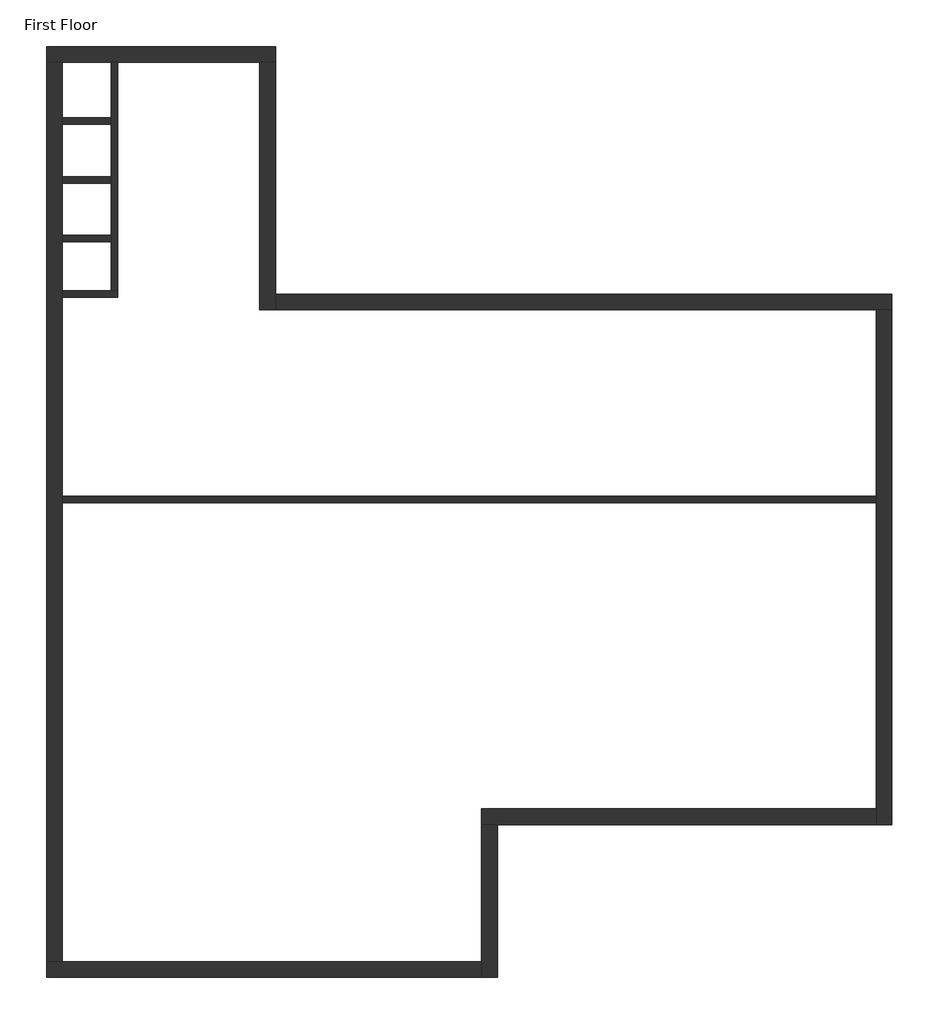
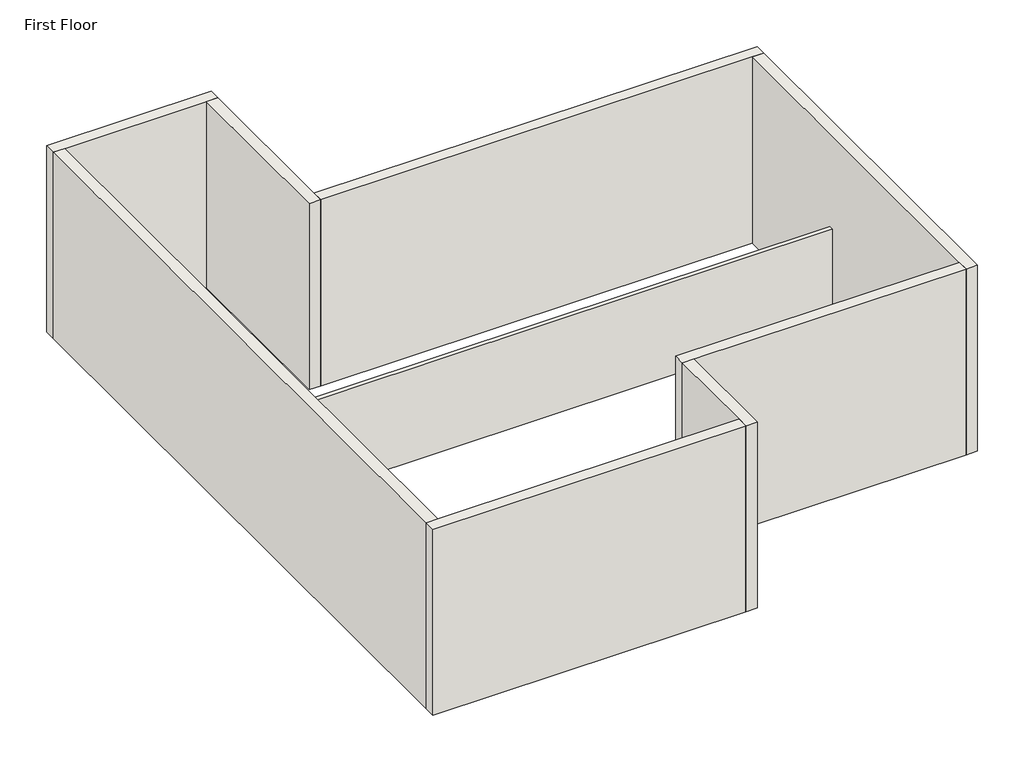
# One storey: 14 walls.
"""IFC4 building model written with IfcOpenShell, lengths in millimetres."""

from ifc_helpers import new_model, si_unit, origin, origin_with_axes, place, context, project, spatial, polyline, outline, extrude, faceted_brep, element, save

model = new_model("IFC4")

# Units and contexts
model_context = context("Model", 3, world=origin())
ifc_project = project(units=[si_unit("LENGTHUNIT", "METRE", prefix="MILLI")], contexts=[model_context])

# Site, building, storey
site = spatial("IfcSite", under=ifc_project)
building = spatial("IfcBuilding", under=site)
storey = spatial("IfcBuildingStorey", under=building, Name="First Floor", Elevation=0.0)

# Walls
placement = place(None, origin())
element("IfcWall", 1, ObjectType="Exterior - Brick on Wood Stud", at=placement, inside=storey, context=model_context, shape_type="Brep", body=[
    faceted_brep([(-11220.7128554, 8382.2404543, 0.0), (-10938.1378554, 8382.2404543, 0.0), (-10069.7753554, 8382.2404543, 0.0), (-9955.4753554, 8382.2404543, 0.0), (-7421.8253554, 8382.2404543, 0.0), (-7139.2503554, 8382.2404543, 0.0), (-7139.2503554, 8382.2404543, 4876.8), (-7421.8253554, 8382.2404543, 4876.8), (-10938.1378554, 8382.2404543, 4876.8), (-11220.7128554, 8382.2404543, 4876.8), (-11220.7128554, 8664.8154543, 0.0), (-11220.7128554, 8664.8154543, 4876.8), (-7139.2503554, 8664.8154543, 4876.8), (-7139.2503554, 8664.8154543, 0.0)], [[[0, 1, 2, 3, 4, 5, 6, 7, 8, 9]], [[10, 11, 12, 13]], [[5, 4, 3, 2, 1, 0, 10, 13]], [[9, 8, 7, 6, 12, 11]], [[6, 5, 13, 12]], [[0, 9, 11, 10]]]),
])
element("IfcWall", 2, ObjectType="Exterior - Brick on Wood Stud", at=placement, inside=storey, context=model_context, shape_type="Brep", body=[
    faceted_brep([(-7421.8253554, 8382.2404543, 0.0), (-7421.8253554, 3973.7529543, 0.0), (-7421.8253554, 3973.7529543, 4876.8), (-7421.8253554, 8382.2404543, 4876.8), (-7139.2503554, 8382.2404543, 0.0), (-7139.2503554, 8382.2404543, 4876.8), (-7139.2503554, 4256.3279543, 4876.8), (-7139.2503554, 3973.7529543, 4876.8), (-7139.2503554, 3973.7529543, 0.0), (-7139.2503554, 4256.3279543, 0.0)], [[[0, 1, 2, 3]], [[4, 5, 6, 7, 8, 9]], [[1, 0, 4, 9, 8]], [[3, 2, 7, 6, 5]], [[0, 3, 5, 4]], [[2, 1, 8, 7]]]),
])
element("IfcWall", 3, ObjectType="Exterior - Brick on Wood Stud", at=placement, inside=storey, context=model_context, shape_type="Brep", body=[
    faceted_brep([(-7139.2503554, 3973.7529543, 0.0), (3562.0871446, 3973.7529543, 0.0), (3844.6621446, 3973.7529543, 0.0), (3844.6621446, 3973.7529543, 4876.8), (3562.0871446, 3973.7529543, 4876.8), (-7139.2503554, 3973.7529543, 4876.8), (-7139.2503554, 4256.3279543, 0.0), (-7139.2503554, 4256.3279543, 4876.8), (3844.6621446, 4256.3279543, 4876.8), (3844.6621446, 4256.3279543, 0.0)], [[[0, 1, 2, 3, 4, 5]], [[6, 7, 8, 9]], [[2, 1, 0, 6, 9]], [[5, 4, 3, 8, 7]], [[0, 5, 7, 6]], [[3, 2, 9, 8]]]),
])
element("IfcWall", 4, ObjectType="Exterior - Brick on Wood Stud", at=placement, inside=storey, context=model_context, shape_type="Brep", body=[
    faceted_brep([(3562.0871446, 3973.7529543, 0.0), (3562.0871446, 655.8779543, 0.0), (3562.0871446, 541.5779543, 0.0), (3562.0871446, -4909.8970457, 0.0), (3562.0871446, -5192.4720457, 0.0), (3562.0871446, -5192.4720457, 4876.8), (3562.0871446, -4909.8970457, 4876.8), (3562.0871446, 3973.7529543, 4876.8), (3844.6621446, 3973.7529543, 0.0), (3844.6621446, 3973.7529543, 4876.8), (3844.6621446, -5192.4720457, 4876.8), (3844.6621446, -5192.4720457, 0.0)], [[[0, 1, 2, 3, 4, 5, 6, 7]], [[8, 9, 10, 11]], [[4, 3, 2, 1, 0, 8, 11]], [[7, 6, 5, 10, 9]], [[0, 7, 9, 8]], [[5, 4, 11, 10]]]),
])
element("IfcWall", 5, ObjectType="Exterior - Brick on Wood Stud", at=placement, inside=storey, context=model_context, shape_type="Brep", body=[
    faceted_brep([(3562.0871446, -4909.8970457, 0.0), (-3470.5378554, -4909.8970457, 0.0), (-3470.5378554, -4909.8970457, 4876.8), (3562.0871446, -4909.8970457, 4876.8), (3562.0871446, -5192.4720457, 0.0), (3562.0871446, -5192.4720457, 4876.8), (-3187.9628554, -5192.4720457, 4876.8), (-3470.5378554, -5192.4720457, 4876.8), (-3470.5378554, -5192.4720457, 0.0), (-3187.9628554, -5192.4720457, 0.0)], [[[0, 1, 2, 3]], [[4, 5, 6, 7, 8, 9]], [[1, 0, 4, 9, 8]], [[3, 2, 7, 6, 5]], [[0, 3, 5, 4]], [[2, 1, 8, 7]]]),
])
element("IfcWall", 6, ObjectType="Exterior - Brick on Wood Stud", at=placement, inside=storey, context=model_context, shape_type="Brep", body=[
    faceted_brep([(-3470.5378554, -5192.4720457, 0.0), (-3470.5378554, -7630.8720457, 0.0), (-3470.5378554, -7913.4470457, 0.0), (-3470.5378554, -7913.4470457, 4876.8), (-3470.5378554, -7630.8720457, 4876.8), (-3470.5378554, -5192.4720457, 4876.8), (-3187.9628554, -5192.4720457, 0.0), (-3187.9628554, -5192.4720457, 4876.8), (-3187.9628554, -7913.4470457, 4876.8), (-3187.9628554, -7913.4470457, 0.0)], [[[0, 1, 2, 3, 4, 5]], [[6, 7, 8, 9]], [[2, 1, 0, 6, 9]], [[5, 4, 3, 8, 7]], [[0, 5, 7, 6]], [[3, 2, 9, 8]]]),
])
element("IfcWall", 7, ObjectType="Exterior - Brick on Wood Stud", at=placement, inside=storey, context=model_context, shape_type="Brep", body=[
    faceted_brep([(-3470.5378554, -7630.8720457, 0.0), (-10938.1378554, -7630.8720457, 0.0), (-11220.7128554, -7630.8720457, 0.0), (-11220.7128554, -7630.8720457, 4876.8), (-10938.1378554, -7630.8720457, 4876.8), (-3470.5378554, -7630.8720457, 4876.8), (-3470.5378554, -7913.4470457, 0.0), (-3470.5378554, -7913.4470457, 4876.8), (-11220.7128554, -7913.4470457, 4876.8), (-11220.7128554, -7913.4470457, 0.0)], [[[0, 1, 2, 3, 4, 5]], [[6, 7, 8, 9]], [[2, 1, 0, 6, 9]], [[5, 4, 3, 8, 7]], [[0, 5, 7, 6]], [[3, 2, 9, 8]]]),
])
element("IfcWall", 8, ObjectType="Exterior - Brick on Wood Stud", at=placement, inside=storey, context=model_context, shape_type="Brep", body=[
    faceted_brep([(-10938.1378554, -7630.8720457, 0.0), (-10938.1378554, 541.5779543, 0.0), (-10938.1378554, 655.8779543, 0.0), (-10938.1378554, 4199.1779543, 0.0), (-10938.1378554, 4313.4779543, 0.0), (-10938.1378554, 5187.7935793, 0.0), (-10938.1378554, 5302.0935793, 0.0), (-10938.1378554, 6233.5592043, 0.0), (-10938.1378554, 6347.8592043, 0.0), (-10938.1378554, 7279.3248293, 0.0), (-10938.1378554, 7393.6248293, 0.0), (-10938.1378554, 8382.2404543, 0.0), (-10938.1378554, 8382.2404543, 4876.8), (-10938.1378554, -7630.8720457, 4876.8), (-11220.7128554, -7630.8720457, 0.0), (-11220.7128554, -7630.8720457, 4876.8), (-11220.7128554, 8382.2404543, 4876.8), (-11220.7128554, 8382.2404543, 0.0)], [[[0, 1, 2, 3, 4, 5, 6, 7, 8, 9, 10, 11, 12, 13]], [[14, 15, 16, 17]], [[11, 10, 9, 8, 7, 6, 5, 4, 3, 2, 1, 0, 14, 17]], [[13, 12, 16, 15]], [[0, 13, 15, 14]], [[12, 11, 17, 16]]]),
])
element("IfcWall", 9, ObjectType="Interior - 4 1/2\" Partition", at=placement, inside=storey, context=model_context, shape_type="SweptSolid", body=[
    extrude(outline(polyline([(3562.0871446, 541.5779543), (-10938.1378554, 541.5779543), (-10938.1378554, 655.8779543), (3562.0871446, 655.8779543), (3562.0871446, 541.5779543)])), origin_with_axes(), (0.0, 0.0, 1.0), 2438.4),
])
element("IfcWall", 10, ObjectType="Interior - 4 1/2\" Partition", at=placement, inside=storey, context=model_context, shape_type="Brep", body=[
    faceted_brep([(-10938.1378554, 4199.1779543, 0.0), (-9955.4753554, 4199.1779543, 0.0), (-9955.4753554, 4199.1779543, 2438.4), (-10938.1378554, 4199.1779543, 2438.4), (-10938.1378554, 4313.4779543, 0.0), (-10938.1378554, 4313.4779543, 2438.4), (-10069.7753554, 4313.4779543, 2438.4), (-9955.4753554, 4313.4779543, 2438.4), (-9955.4753554, 4313.4779543, 0.0), (-10069.7753554, 4313.4779543, 0.0)], [[[0, 1, 2, 3]], [[4, 5, 6, 7, 8, 9]], [[1, 0, 4, 9, 8]], [[3, 2, 7, 6, 5]], [[0, 3, 5, 4]], [[2, 1, 8, 7]]]),
])
element("IfcWall", 11, ObjectType="Interior - 4 1/2\" Partition", at=placement, inside=storey, context=model_context, shape_type="Brep", body=[
    faceted_brep([(-9955.4753554, 4313.4779543, 0.0), (-9955.4753554, 8382.2404543, 0.0), (-9955.4753554, 8382.2404543, 2438.4), (-9955.4753554, 4313.4779543, 2438.4), (-10069.7753554, 4313.4779543, 0.0), (-10069.7753554, 4313.4779543, 2438.4), (-10069.7753554, 5187.7935793, 2438.4), (-10069.7753554, 5302.0935793, 2438.4), (-10069.7753554, 6233.5592043, 2438.4), (-10069.7753554, 6347.8592043, 2438.4), (-10069.7753554, 7279.3248293, 2438.4), (-10069.7753554, 7393.6248293, 2438.4), (-10069.7753554, 8382.2404543, 2438.4), (-10069.7753554, 8382.2404543, 0.0), (-10069.7753554, 7393.6248293, 0.0), (-10069.7753554, 7279.3248293, 0.0), (-10069.7753554, 6347.8592043, 0.0), (-10069.7753554, 6233.5592043, 0.0), (-10069.7753554, 5302.0935793, 0.0), (-10069.7753554, 5187.7935793, 0.0)], [[[0, 1, 2, 3]], [[4, 5, 6, 7, 8, 9, 10, 11, 12, 13, 14, 15, 16, 17, 18, 19]], [[1, 0, 4, 19, 18, 17, 16, 15, 14, 13]], [[3, 2, 12, 11, 10, 9, 8, 7, 6, 5]], [[0, 3, 5, 4]], [[2, 1, 13, 12]]]),
])
element("IfcWall", 12, ObjectType="Interior - 4 1/2\" Partition", at=placement, inside=storey, context=model_context, shape_type="SweptSolid", body=[
    extrude(outline(polyline([(-10069.7753554, 5187.7935793), (-10938.1378554, 5187.7935793), (-10938.1378554, 5302.0935793), (-10069.7753554, 5302.0935793), (-10069.7753554, 5187.7935793)])), origin_with_axes(), (0.0, 0.0, 1.0), 2438.4),
])
element("IfcWall", 13, ObjectType="Interior - 4 1/2\" Partition", at=placement, inside=storey, context=model_context, shape_type="SweptSolid", body=[
    extrude(outline(polyline([(-10069.7753554, 6233.5592043), (-10938.1378554, 6233.5592043), (-10938.1378554, 6347.8592043), (-10069.7753554, 6347.8592043), (-10069.7753554, 6233.5592043)])), origin_with_axes(), (0.0, 0.0, 1.0), 2438.4),
])
element("IfcWall", 14, ObjectType="Interior - 4 1/2\" Partition", at=placement, inside=storey, context=model_context, shape_type="SweptSolid", body=[
    extrude(outline(polyline([(-10069.7753554, 7279.3248293), (-10938.1378554, 7279.3248293), (-10938.1378554, 7393.6248293), (-10069.7753554, 7393.6248293), (-10069.7753554, 7279.3248293)])), origin_with_axes(), (0.0, 0.0, 1.0), 2438.4),
])

save(model, "model.ifc")

# Revit data of these elements
# Project information
#   Project Issue Date = "Issue Date"
#   Project Status = "Project Status"
#   Client Name = "Owner"
#   Project Address = "Enter address here"
#   Project Name = "Project Name"
#   Project Number = "Project Number"
# Grids (mm)
#   "1": line (-10938.138, -13775.472) -> (-10938.138, 9288.695)
#   "2": line (-7280.538, -13775.472) -> (-7280.538, 9288.695)
#   "3": line (-3470.538, -13775.472) -> (-3470.538, 9288.695)
#   "4": line (187.062, -13775.472) -> (187.062, 9288.695)
#   "5": line (3844.662, -13775.472) -> (3844.662, 9288.695)
#   "B": line (6207.412, 4256.328) -> (-13740.722, 4256.328)
#   "C": line (6207.412, 598.728) -> (-13740.722, 598.728)
#   "D": line (6207.412, -3058.872) -> (-13740.722, -3058.872)
#   "D.1": line (6207.412, -5192.472) -> (-13740.722, -5192.472)
#   "E": line (6207.412, -7630.872) -> (-13740.722, -7630.872)
#   "F": line (6207.412, -11898.072) -> (-13740.722, -11898.072)
#   "A": line (6207.412, 7913.928) -> (-13740.722, 7913.928)
# Type "Exterior - Brick on Wood Stud"
#   Assembly Code = "B2010158"
#   Layers, outside or top first: 0' - 3 5/8" "Brick, Common" (function 4); 0' - 1" "Air" (function 3); 0' - 0" "Air Infiltration Barrier" (function 100); 0' - 0 1/2" "Plywood, Sheathing" (function 2); 0' - 5 1/2" "Softwood, Lumber" (function 1); 0' - 0" "Vapor Retarder" (function 100); 0' - 0 1/2" "Gypsum Wall Board" (function 5)
# Type "Interior - 4 1/2\" Partition"
#   Assembly Code = "C1010145"
#   Layers, outside or top first: 0' - 0 1/2" "Gypsum Wall Board" (function 5); 0' - 3 1/2" "Softwood, Lumber" (function 1); 0' - 0 1/2" "Gypsum Wall Board" (function 5)
# Element 1 (IfcWall, "Exterior - Brick on Wood Stud")
#   Top Offset = 0' - 0"
#   Base Offset = 0' - 0"
#   wall height = 16' - 0"
#   Phase Created = New Construction
#   Base Constraint = First Floor
#   Top Constraint = Roof
#   Materials on its faces: "Brick, Common", "Default Wall", "Gypsum Wall Board"
# Elements 2, 5, 8 (IfcWall, "Exterior - Brick on Wood Stud")
#   Top Offset = 0' - 0"
#   Base Offset = 0' - 0"
#   wall height = 16' - 0"
#   Phase Created = New Construction
#   Base Constraint = First Floor
#   Top Constraint = Roof
#   Materials on its faces: "Default Wall", "Gypsum Wall Board", "Brick, Common"
# Elements 3, 4, 6, 7 (IfcWall, "Exterior - Brick on Wood Stud")
#   Top Offset = 0' - 0"
#   Base Offset = 0' - 0"
#   wall height = 16' - 0"
#   Phase Created = New Construction
#   Base Constraint = First Floor
#   Top Constraint = Roof
#   Materials on its faces: "Default Wall", "Brick, Common", "Gypsum Wall Board"
# Elements 9, 11, 12, 13, 14 (IfcWall, "Interior - 4 1/2\" Partition")
#   Top Offset = 0' - 0"
#   Base Offset = 0' - 0"
#   Unconnected Height = 8' - 0"
#   wall height = 8' - 0"
#   Phase Created = New Construction
#   Base Constraint = First Floor
#   Materials on its faces: "Default Wall", "Gypsum Wall Board"
# Element 10 (IfcWall, "Interior - 4 1/2\" Partition")
#   Top Offset = 0' - 0"
#   Base Offset = 0' - 0"
#   Unconnected Height = 8' - 0"
#   wall height = 8' - 0"
#   Phase Created = New Construction
#   Base Constraint = First Floor
#   Materials on its faces: "Gypsum Wall Board", "Default Wall"
# Materials
#   "Brick, Common": class "Masonry", colour RGB 85 47 55, transparency 0, Description = "Common brick", Cost = 0
#   "Air": class "Gas", colour RGB 229 229 229, transparency 1, Description = "Air", Cost = 0
#   "Air Infiltration Barrier": class "Generic", colour RGB 80 80 80, transparency 0, Description = "physical material", Cost = 0
#   "Plywood, Sheathing": class "Wood", colour RGB 193 140 64, transparency 0, Description = "Plywood, sheathing grade", Cost = 0
#   "Softwood, Lumber": class "Wood", colour RGB 234 198 147, transparency 0, Description = "Pinus Echinata", Cost = 0
#   "Vapor Retarder": class "Generic", colour RGB 80 80 80, transparency 0, Description = "Polyethylene film membrane", Cost = 0
#   "Gypsum Wall Board": class "Generic", colour RGB 228 228 228, transparency 0, Description = "Gypsum Wall Board", Cost = 0
#   "Default Wall": class "Miscellaneous", colour RGB 80 80 80, transparency 0, Cost = 0
